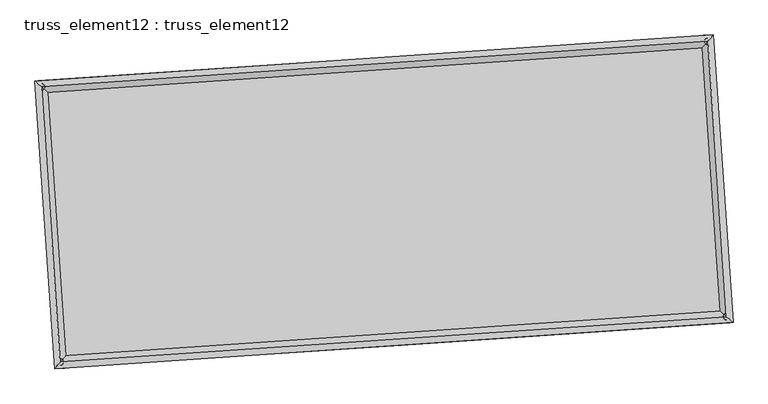
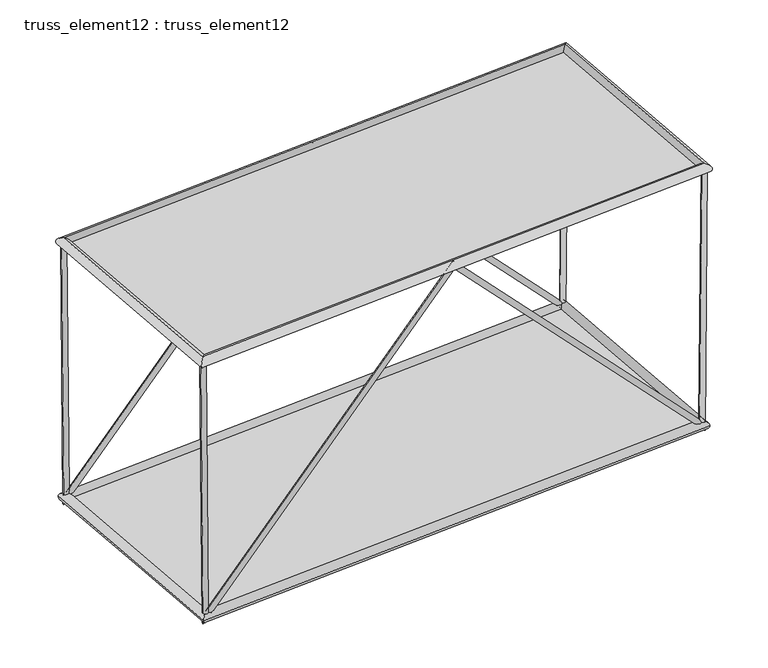
"""IFC4 building model written with IfcOpenShell, lengths in millimetres: plate geometry, truss_element12 : truss_element12."""

from ifc_helpers import new_model, si_unit, frame, origin, origin_with_axes, place, context, project, spatial, polyline, circle_curve, ellipse_curve, outline, extrude, source, transform, mapped, element, save
from ifc_brep_helpers import plane_surface, cylinder_surface, advanced_brep


def truss_element12_truss_element12_f6fe5973(model_context):
    return source(origin(), model_context, "Body", "SolidModel", [
        advanced_brep(
        [(-3710.2419701, 2273.1351163, 5000.2468963), (-3809.3412307, 2259.7741453, 4999.3408025), (-3666.054382, 2276.1481, 123.0325372), (-3762.9325009, 2262.9385801, -123.0325372), (1064.1133725, 2598.6802581, 5071.9126382), (1064.5556921, 2592.106649, 4927.6678811), (5793.5123498, 2921.1599962, 123.0270149), (5891.2486273, 2921.2204923, -123.0270149), (5838.4629041, 2924.2250036, 5000.2475381), (5938.4584258, 2924.439549, 4999.3258017)],
        [
            (0, 1, circle_curve(frame((-3759.7916004, 2266.4546308, 4999.7938494), z_axis=(-0.009059631795656001, -0.0006177418532641554, 0.9999587698834037), x_axis=(-0.13360979880213997, 0.991033835814136, -0.0005982771700932393)), 50.0)),
            (1, 0, circle_curve(frame((-3759.7916004, 2266.4546308, 4999.7938494), z_axis=(-0.009059631795656001, -0.0006177418532641554, 0.9999587698834037), x_axis=(-0.13360979880213997, 0.991033835814136, -0.0005982771700932393)), 50.0)),
            (0, 2),
            (2, 3, ellipse_curve(frame((-3714.4934414, 2269.54334, 0.0), z_axis=(-0.9274570070583217, -0.06323976771716287, 0.3685433920686947), x_axis=(0.36768962300005015, 0.02507135767326109, 0.9296105464991781)), 132.6366613, 50.0)),
            (3, 1),
            (3, 2, ellipse_curve(frame((-3714.4934414, 2269.54334, 0.0), z_axis=(-0.9274570070583217, -0.06323976771716287, 0.3685433920686947), x_axis=(0.36768962300005015, 0.02507135767326109, 0.9296105464991781)), 132.6366613, 50.0)),
            (2, 4),
            (4, 5, ellipse_curve(frame((1064.3345323, 2595.3934535, 4999.7902597), z_axis=(-0.9976833952413823, -0.06802823817187122, 4.0876142565046614e-05), x_axis=(-4.078144873295169e-05, -2.7807319613378337e-06, -0.9999999991645705)), 72.2794243, 50.0)),
            (5, 3),
            (5, 4, ellipse_curve(frame((1064.3345323, 2595.3934535, 4999.7902597), z_axis=(-0.9976833952413823, -0.06802823817187122, 4.0876142565046614e-05), x_axis=(-4.078144873295169e-05, -2.7807319613378337e-06, -0.9999999991645705)), 72.2794243, 50.0)),
            (4, 6),
            (6, 7, ellipse_curve(frame((5842.3804885, 2921.1902443, 0.0), z_axis=(-0.9275008521416513, -0.06324275734672206, -0.3684325215282904), x_axis=(-0.36757900930277465, -0.025063815345731454, 0.9296544933900474)), 132.6244381, 50.0)),
            (7, 5),
            (7, 6, ellipse_curve(frame((5842.3804885, 2921.1902443, 0.0), z_axis=(-0.9275008521416513, -0.06324275734672206, -0.3684325215282904), x_axis=(-0.36757900930277465, -0.025063815345731454, 0.9296544933900474)), 132.6244381, 50.0)),
            (8, 9, circle_curve(frame((5888.4606649, 2924.3322763, 4999.7866699), z_axis=(0.009216035288573994, 0.0006284064128948841, 0.9999573339892758), x_axis=(-0.0021511542640449003, 0.9999975010640975, -0.0006086056957160734)), 50.0)),
            (9, 8, circle_curve(frame((5888.4606649, 2924.3322763, 4999.7866699), z_axis=(0.009216035288573994, 0.0006284064128948841, 0.9999573339892758), x_axis=(-0.0021511542640449003, 0.9999975010640975, -0.0006086056957160734)), 50.0)),
            (6, 8),
            (9, 7),
        ],
        [
            plane_surface(frame((-3759.7916004, 2316.4546212, 4999.8247378), z_axis=(-0.00905963179565723, -0.0006177418532678904, 0.9999587698834038), x_axis=(0.9999589606937513, -5.596743421598659e-06, 0.00905963006691479))),
            cylinder_surface(frame((-3759.7916004, 2266.4546308, 4999.7938494), z_axis=(-0.009059631795656003, -0.0006177418532641555, 0.9999587698834039), x_axis=(-0.13360979880213997, 0.991033835814136, -0.0005982771700932393)), 50.0),
            cylinder_surface(frame((-3714.4934414, 2269.54334, 0.0), z_axis=(-0.6901867139153417, -0.04706120837656332, -0.7220993993910259), x_axis=(-0.020415334139245483, 0.9987521360670553, -0.0455783373268222)), 50.0),
            cylinder_surface(frame((1064.3345323, 2595.3934535, 4999.7902597), z_axis=(-0.6901278150897087, -0.047057192289543075, 0.7221559523353178), x_axis=(-0.11534924188526842, 0.9922789537754221, -0.04557444778434232)), 50.0),
            plane_surface(frame((5888.4606649, 2874.3322862, 4999.8180916), z_axis=(0.009216035288575347, 0.0006284064128996202, 0.9999573339892759), x_axis=(0.9999575314449909, -5.7916616409414675e-06, -0.009216033468739223))),
            cylinder_surface(frame((5842.3804885, 2921.1902443, 0.0), z_axis=(-0.009216035288573994, -0.0006284064128948841, -0.9999573339892758), x_axis=(-0.0021511542640449003, 0.9999975010640975, -0.0006086056957160734)), 50.0),
        ],
        [
            (0, [[1, 2]]),
            (1, [[-1, 3, 4, 5]]),
            (1, [[-2, -5, 6, -3]]),
            (2, [[-4, 7, 8, 9]]),
            (2, [[-6, -9, 10, -7]]),
            (3, [[-8, 11, 12, 13]]),
            (3, [[-10, -13, 14, -11]]),
            (4, [[15, 16]]),
            (5, [[-12, 17, -16, 18]]),
            (5, [[-14, -18, -15, -17]]),
        ],
    ),
        advanced_brep(
        [(-3438.1290172, -1717.598468, 5000.2468963), (-3537.2282778, -1730.959439, 4999.3408025), (-3393.941429, -1714.5854843, 123.0325372), (-3490.819548, -1727.7950042, -123.0325372), (1336.2263254, -1392.0533262, 5071.9126382), (1336.668645, -1398.6269353, 4927.6678811), (6065.6253027, -1069.5735881, 123.0270149), (6163.3615802, -1069.513092, -123.0270149), (6110.575857, -1066.5085807, 5000.2475381), (6210.5713787, -1066.2940353, 4999.3258017)],
        [
            (0, 1, circle_curve(frame((-3487.6786475, -1724.2789535, 4999.7938494), z_axis=(-0.009059631795655944, -0.0006177418532642077, 0.9999587698834038), x_axis=(-0.13360979880213966, 0.991033835814136, -0.0005982771700931769)), 50.0)),
            (1, 0, circle_curve(frame((-3487.6786475, -1724.2789535, 4999.7938494), z_axis=(-0.009059631795655944, -0.0006177418532642077, 0.9999587698834038), x_axis=(-0.13360979880213966, 0.991033835814136, -0.0005982771700931769)), 50.0)),
            (0, 2),
            (2, 3, ellipse_curve(frame((-3442.3804885, -1721.1902443, 0.0), z_axis=(-0.9274570070583221, -0.06323976771716276, 0.3685433920686939), x_axis=(0.3676896230000495, 0.025071357673260925, 0.9296105464991783)), 132.6366613, 50.0)),
            (3, 1),
            (3, 2, ellipse_curve(frame((-3442.3804885, -1721.1902443, 0.0), z_axis=(-0.9274570070583221, -0.06323976771716276, 0.3685433920686939), x_axis=(0.3676896230000495, 0.025071357673260925, 0.9296105464991783)), 132.6366613, 50.0)),
            (2, 4),
            (4, 5, ellipse_curve(frame((1336.4474852, -1395.3401308, 4999.7902597), z_axis=(-0.9976833952413823, -0.06802823817187109, 4.0876142564083687e-05), x_axis=(-4.07814487320292e-05, -2.7807319611648704e-06, -0.9999999991645705)), 72.2794243, 50.0)),
            (5, 3),
            (5, 4, ellipse_curve(frame((1336.4474852, -1395.3401308, 4999.7902597), z_axis=(-0.9976833952413823, -0.06802823817187109, 4.0876142564083687e-05), x_axis=(-4.07814487320292e-05, -2.7807319611648704e-06, -0.9999999991645705)), 72.2794243, 50.0)),
            (4, 6),
            (6, 7, ellipse_curve(frame((6114.4934414, -1069.54334, 0.0), z_axis=(-0.9275008521416513, -0.06324275734672197, -0.3684325215282904), x_axis=(-0.36757900930277465, -0.02506381534573148, 0.9296544933900474)), 132.6244381, 50.0)),
            (7, 5),
            (7, 6, ellipse_curve(frame((6114.4934414, -1069.54334, 0.0), z_axis=(-0.9275008521416513, -0.06324275734672197, -0.3684325215282904), x_axis=(-0.36757900930277465, -0.02506381534573148, 0.9296544933900474)), 132.6244381, 50.0)),
            (8, 9, circle_curve(frame((6160.5736179, -1066.401308, 4999.7866699), z_axis=(0.009216035288574044, 0.0006284064128948374, 0.9999573339892759), x_axis=(-0.0021511542640451015, 0.9999975010640975, -0.0006086056957160248)), 50.0)),
            (9, 8, circle_curve(frame((6160.5736179, -1066.401308, 4999.7866699), z_axis=(0.009216035288574044, 0.0006284064128948374, 0.9999573339892759), x_axis=(-0.0021511542640451015, 0.9999975010640975, -0.0006086056957160248)), 50.0)),
            (6, 8),
            (9, 7),
        ],
        [
            plane_surface(frame((-3487.6786475, -1674.2789631, 4999.8247378), z_axis=(-0.00905963179565723, -0.0006177418532678904, 0.9999587698834038), x_axis=(0.9999589606937513, -5.596743421598659e-06, 0.00905963006691479))),
            cylinder_surface(frame((-3487.6786475, -1724.2789535, 4999.7938494), z_axis=(-0.009059631795655944, -0.0006177418532642077, 0.9999587698834038), x_axis=(-0.13360979880213966, 0.991033835814136, -0.0005982771700931769)), 50.0),
            cylinder_surface(frame((-3442.3804885, -1721.1902443, 0.0), z_axis=(-0.6901867139153405, -0.04706120837656307, -0.7220993993910272), x_axis=(-0.02041533413924536, 0.9987521360670553, -0.04557833732682192)), 50.0),
            cylinder_surface(frame((1336.4474852, -1395.3401308, 4999.7902597), z_axis=(-0.6901278150897087, -0.047057192289543054, 0.7221559523353177), x_axis=(-0.11534924188526818, 0.992278953775422, -0.04557444778434213)), 50.0),
            plane_surface(frame((6160.5736179, -1116.4012981, 4999.8180916), z_axis=(0.009216035288575347, 0.000628406412899621, 0.9999573339892759), x_axis=(0.9999575314449909, -5.791661640497378e-06, -0.009216033468739223))),
            cylinder_surface(frame((6114.4934414, -1069.54334, 0.0), z_axis=(-0.009216035288574044, -0.0006284064128948374, -0.9999573339892759), x_axis=(-0.0021511542640451015, 0.9999975010640975, -0.0006086056957160248)), 50.0),
        ],
        [
            (0, [[1, 2]]),
            (1, [[-1, 3, 4, 5]]),
            (1, [[-2, -5, 6, -3]]),
            (2, [[-4, 7, 8, 9]]),
            (2, [[-6, -9, 10, -7]]),
            (3, [[-8, 11, 12, 13]]),
            (3, [[-10, -13, 14, -11]]),
            (4, [[15, 16]]),
            (5, [[-12, 17, -16, 18]]),
            (5, [[-14, -18, -15, -17]]),
        ],
    ),
        advanced_brep(
        [(-3487.6805382, -1724.2810491, 4909.7938494), (-3487.6767568, -1724.276858, 5089.7938494), (-3759.7894427, 2266.4528113, 5089.7938494), (-3759.7937581, 2266.4564503, 4909.7938494), (5888.4589075, 2924.3301899, 5089.7866699), (5888.4624223, 2924.3343628, 4909.78667), (6160.5715935, -1066.3994794, 5089.7866699), (6160.5756422, -1066.4031366, 4909.78667)],
        [
            (0, 1, ellipse_curve(frame((-3487.6786475, -1724.2789535, 4999.7938494), z_axis=(-0.7535719234052624, 0.6573654662780954, 5.249543265090631e-07), x_axis=(-0.6573654662778877, -0.7535719234054434, 5.249543265091374e-07)), 127.2792206, 90.0)),
            (1, 2),
            (2, 3, ellipse_curve(frame((-3759.7916004, 2266.4546308, 4999.7938494), z_axis=(-0.6573654662778875, -0.7535719234054435, 5.249543277760535e-07), x_axis=(0.7535719234052622, -0.6573654662780956, -5.249543277759792e-07)), 127.2792206, 90.0)),
            (3, 0),
            (1, 0, ellipse_curve(frame((-3487.6786475, -1724.2789535, 4999.7938494), z_axis=(-0.7535719234052624, 0.6573654662780954, 5.249543265090631e-07), x_axis=(-0.6573654662778877, -0.7535719234054434, 5.249543265091374e-07)), 127.2792206, 90.0)),
            (3, 2, ellipse_curve(frame((-3759.7916004, 2266.4546308, 4999.7938494), z_axis=(-0.6573654662778875, -0.7535719234054435, 5.249543277760535e-07), x_axis=(0.7535719234052622, -0.6573654662780956, -5.249543277759792e-07)), 127.2792206, 90.0)),
            (2, 4),
            (4, 5, ellipse_curve(frame((5888.4606649, 2924.3322763, 4999.7866699), z_axis=(-0.7535719234052609, 0.6573654662780971, 5.2495432471324e-07), x_axis=(-0.6573654662778895, -0.7535719234054419, 5.249543308387929e-07)), 127.2792206, 90.0)),
            (5, 3),
            (5, 4, ellipse_curve(frame((5888.4606649, 2924.3322763, 4999.7866699), z_axis=(-0.7535719234052609, 0.6573654662780971, 5.2495432471324e-07), x_axis=(-0.6573654662778895, -0.7535719234054419, 5.249543308387929e-07)), 127.2792206, 90.0)),
            (4, 6),
            (6, 7, ellipse_curve(frame((6160.5736179, -1066.401308, 4999.7866699), z_axis=(0.6573654662778894, 0.753571923405442, -5.249543295718767e-07), x_axis=(-0.7535719234052608, 0.6573654662780972, 5.249543234463237e-07)), 127.2792206, 90.0)),
            (7, 5),
            (7, 6, ellipse_curve(frame((6160.5736179, -1066.401308, 4999.7866699), z_axis=(0.6573654662778894, 0.753571923405442, -5.249543295718767e-07), x_axis=(-0.7535719234052608, 0.6573654662780972, 5.249543234463237e-07)), 127.2792206, 90.0)),
            (6, 1),
            (0, 7),
        ],
        [
            cylinder_surface(frame((-3487.6786475, -1724.2789535, 4999.7938494), z_axis=(0.06802823822869923, -0.9976833960748769, 0.0), x_axis=(-0.9976833958213659, -0.06802823821141327, 2.254327394957503e-05)), 90.0),
            cylinder_surface(frame((-3759.7916004, 2266.4546308, 4999.7938494), z_axis=(-0.9976833960746017, -0.06802823822868122, 7.423975299672935e-07), x_axis=(-0.06802823819638637, 0.9976833958388891, 2.1800876419784193e-05)), 90.0),
            cylinder_surface(frame((5888.4606649, 2924.3322763, 4999.7866699), z_axis=(-0.0680282382286945, 0.9976833960748772, 0.0), x_axis=(0.9976833958536611, 0.0680282382136106, 2.1058478894324835e-05)), 90.0),
            cylinder_surface(frame((6160.5736179, -1066.401308, 4999.7866699), z_axis=(0.9976833960746018, 0.06802823822868093, -7.423975281756036e-07), x_axis=(0.06802823822868093, -0.9976833958366871, 2.180087642665553e-05)), 90.0),
        ],
        [
            (0, [[1, 2, 3, 4]]),
            (0, [[5, -4, 6, -2]]),
            (1, [[-3, 7, 8, 9]]),
            (1, [[-6, -9, 10, -7]]),
            (2, [[-8, 11, 12, 13]]),
            (2, [[-10, -13, 14, -11]]),
            (3, [[-12, 15, -1, 16]]),
            (3, [[-14, -16, -5, -15]]),
        ],
    ),
        advanced_brep(
        [(-3358.7115243, -1625.2761972, 0.0), (-3526.0494527, -1817.1042913, 0.0), (-3810.4074885, 2353.2123043, 0.0), (-3618.5793943, 2185.8743758, 0.0), (5926.0494527, 3017.1042913, 0.0), (5758.7115243, 2825.2761972, 0.0), (6210.4074885, -1153.2123043, 0.0), (6018.5793943, -985.8743758, 0.0)],
        [
            (0, 1, ellipse_curve(frame((-3442.3804885, -1721.1902443, 0.0), z_axis=(-0.7535719234054598, 0.6573654662780787, 0.0), x_axis=(-0.6573654662780787, -0.7535719234054599, 0.0)), 127.2792206, 90.0)),
            (1, 2),
            (2, 3, ellipse_curve(frame((-3714.4934414, 2269.54334, 0.0), z_axis=(-0.6573654662780787, -0.7535719234054599, 0.0), x_axis=(0.7535719234054599, -0.6573654662780785, 0.0)), 127.2792206, 90.0)),
            (3, 0),
            (1, 0, ellipse_curve(frame((-3442.3804885, -1721.1902443, 0.0), z_axis=(-0.7535719234054598, 0.6573654662780787, 0.0), x_axis=(-0.6573654662780787, -0.7535719234054599, 0.0)), 127.2792206, 90.0)),
            (3, 2, ellipse_curve(frame((-3714.4934414, 2269.54334, 0.0), z_axis=(-0.6573654662780787, -0.7535719234054599, 0.0), x_axis=(0.7535719234054599, -0.6573654662780785, 0.0)), 127.2792206, 90.0)),
            (2, 4),
            (4, 5, ellipse_curve(frame((5842.3804885, 2921.1902443, 0.0), z_axis=(-0.7535719234054583, 0.6573654662780803, 0.0), x_axis=(-0.6573654662780803, -0.7535719234054582, 0.0)), 127.2792206, 90.0)),
            (5, 3),
            (5, 4, ellipse_curve(frame((5842.3804885, 2921.1902443, 0.0), z_axis=(-0.7535719234054583, 0.6573654662780803, 0.0), x_axis=(-0.6573654662780803, -0.7535719234054582, 0.0)), 127.2792206, 90.0)),
            (4, 6),
            (6, 7, ellipse_curve(frame((6114.4934414, -1069.54334, 0.0), z_axis=(0.6573654662780805, 0.7535719234054583, 0.0), x_axis=(-0.7535719234054584, 0.6573654662780803, 0.0)), 127.2792206, 90.0)),
            (7, 5),
            (7, 6, ellipse_curve(frame((6114.4934414, -1069.54334, 0.0), z_axis=(0.6573654662780805, 0.7535719234054583, 0.0), x_axis=(-0.7535719234054584, 0.6573654662780803, 0.0)), 127.2792206, 90.0)),
            (6, 1),
            (0, 7),
        ],
        [
            cylinder_surface(frame((-3442.3804885, -1721.1902443, 0.0), z_axis=(0.06802823822870352, -0.9976833960748764, 0.0), x_axis=(-0.9976833960748764, -0.06802823822870352, 0.0)), 90.0),
            cylinder_surface(frame((-3714.4934414, 2269.54334, 0.0), z_axis=(-0.9976833960748764, -0.06802823822870463, 0.0), x_axis=(-0.06802823822870463, 0.9976833960748764, 0.0)), 90.0),
            cylinder_surface(frame((5842.3804885, 2921.1902443, 0.0), z_axis=(-0.0680282382286991, 0.9976833960748769, 0.0), x_axis=(0.9976833960748769, 0.0680282382286991, 0.0)), 90.0),
            cylinder_surface(frame((6114.4934414, -1069.54334, 0.0), z_axis=(0.9976833960748764, 0.06802823822870442, 0.0), x_axis=(0.06802823822870442, -0.9976833960748764, 0.0)), 90.0),
        ],
        [
            (0, [[1, 2, 3, 4]]),
            (0, [[5, -4, 6, -2]]),
            (1, [[-3, 7, 8, 9]]),
            (1, [[-6, -9, 10, -7]]),
            (2, [[-8, 11, 12, 13]]),
            (2, [[-10, -13, 14, -11]]),
            (3, [[-12, 15, -1, 16]]),
            (3, [[-14, -16, -5, -15]]),
        ],
    ),
        extrude(outline(polyline([(-3442.3804885, -1721.1902443), (-3714.4934414, 2269.54334), (5842.3804885, 2921.1902443), (6114.4934414, -1069.54334), (-3442.3804885, -1721.1902443)])), origin_with_axes(), (0.0, 0.0, 1.0), 20.0),
        extrude(outline(polyline([(-2000.0, 4835.3276717), (2000.0, 4835.3276717), (2000.0, -4835.3276717), (-2000.0, -4835.3276718), (-2000.0, 4835.3276717)])), frame((1200.3910087, 600.0266614, 4999.7902597), z_axis=(7.406776889353197e-07, 5.050399602901239e-08, 0.9999999999997244), x_axis=(-0.06802823822870309, 0.9976833960748765, 0.0)), (0.0, 0.0, 1.0), 20.0),
    ])


if __name__ == "__main__":
    model = new_model("IFC4")
    model_context = context("Model", 3, world=origin())
    ifc_project = project(units=[si_unit("LENGTHUNIT", "METRE", prefix="MILLI")], contexts=[model_context])
    site = spatial("IfcSite", under=ifc_project)
    building = spatial("IfcBuilding", under=site)
    placement = place(None, origin())
    truss_element12_truss_element12_shape = truss_element12_truss_element12_f6fe5973(model_context)
    element("IfcPlate", 1, ObjectType="truss_element12 : truss_element12", at=placement, inside=building, context=model_context, shape_type="MappedRepresentation", body=[
        mapped(truss_element12_truss_element12_shape, transform((0.0, 0.0, 0.0), x_axis=(1.0, 0.0, 0.0), y_axis=(0.0, 1.0, 0.0), z_axis=(0.0, 0.0, 1.0))),
    ])
    save(model, "model.ifc")

# Revit data of these elements
# Type "truss_element12 : truss_element12"
#   steellbar1 = 90 mm
#   steelbar2 = 50 mm
#   offset1 = 5000 mm
#   M = Default Roof
# Element 1 (IfcPlate, "truss_element12 : truss_element12")
#   Materials on its faces: "Default Roof"
# Materials
#   "Default Roof": class "Miscellaneous", colour RGB 0 127 0, transparency 0, Comments = "Rendering appearance not upgraded Rendering appearance not upgraded ", Cost = 0
